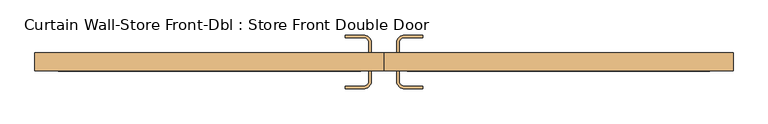
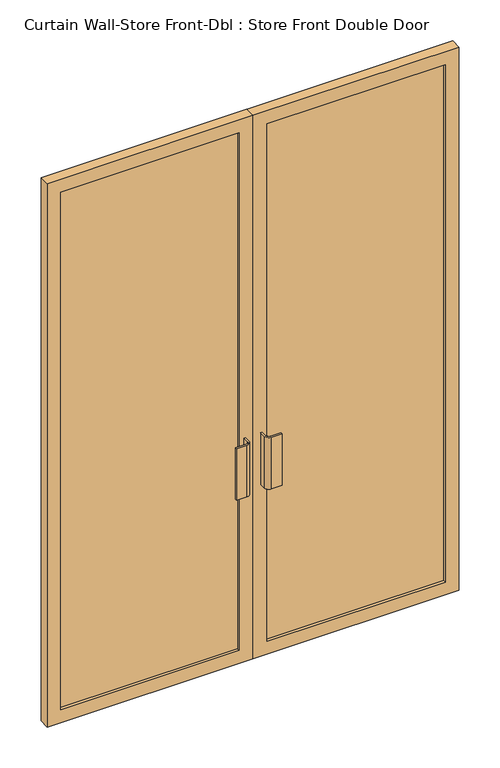
"""IFC4 building model written with IfcOpenShell, lengths in millimetres: door geometry, Curtain Wall-Store Front-Dbl : Store Front Double Door."""

import ifcopenshell
import ifcopenshell.guid

model = None  # the IFC model being written
_history = None  # IfcOwnerHistory: only IFC2X3 demands one
_inside = {}  # id of a spatial element -> (the spatial element, [elements in it])
_under = {}  # id of a project, library or spatial element -> (it, [spatial elements below it])
_declared = {}  # id of a project -> (the project, [libraries it declares])
_typed = {}  # id of a type object -> (the type object, [elements of that type])
_made_of = {}  # id of a material, layer set ... -> (it, [elements and type objects made of it])


def new_model(schema):
    """Start an empty IFC model of exactly this schema.

    Asked for "IFC4X3", IfcOpenShell would pick the latest addendum, in which some entities
    have other attributes; the version numbers below select the first issue.
    IFC2X3 requires an IfcOwnerHistory on every rooted entity: one is made here for all.
    """
    global model, _history
    if schema == "IFC4X3":
        model = ifcopenshell.file(schema_version=(4, 3, 0, 0))
    else:
        model = ifcopenshell.file(schema=schema)
    _inside.clear()
    _under.clear()
    _declared.clear()
    _typed.clear()
    _made_of.clear()
    _history = None
    if model.schema == "IFC2X3":
        org = make("IfcOrganization", Name="unknown")
        user = make(
            "IfcPersonAndOrganization",
            ThePerson=make("IfcPerson", FamilyName="unknown"),
            TheOrganization=org,
        )
        app = make(
            "IfcApplication",
            ApplicationDeveloper=org,
            Version="unknown",
            ApplicationFullName="unknown",
            ApplicationIdentifier="unknown",
        )
        _history = make(
            "IfcOwnerHistory",
            OwningUser=user,
            OwningApplication=app,
            ChangeAction="ADDED",
            CreationDate=0,
        )
    return model


def make(cls, **values):
    """One entity of the class cls with the attributes given. An attribute that is None is left unset."""
    return model.create_entity(
        cls, **{name: value for name, value in values.items() if value is not None}
    )


def rooted(cls, **values):
    """An entity with a GlobalId (a new one), such as an element, a storey or a relation."""
    return make(cls, GlobalId=ifcopenshell.guid.new(), OwnerHistory=_history, **values)


def si_unit(unit_type, name, prefix=None):
    """IfcSIUnit, for example si_unit("LENGTHUNIT", "METRE", prefix="MILLI")."""
    return make("IfcSIUnit", UnitType=unit_type, Prefix=prefix, Name=name)


def assignment(units):
    """IfcUnitAssignment: the units of a project."""
    return None if units is None else make("IfcUnitAssignment", Units=units)


def point(xyz):
    """IfcCartesianPoint."""
    return None if xyz is None else make("IfcCartesianPoint", Coordinates=xyz)


def direction(xyz):
    """IfcDirection."""
    return None if xyz is None else make("IfcDirection", DirectionRatios=xyz)


def frame(location, z_axis=None, x_axis=None):
    """IfcAxis2Placement3D, a coordinate frame: its origin and axes. An axis left out is left unset."""
    return make(
        "IfcAxis2Placement3D",
        Location=point(location),
        Axis=direction(z_axis),
        RefDirection=direction(x_axis),
    )


def frame_2d(location, x_axis=None):
    """IfcAxis2Placement2D, a coordinate frame in the plane: its origin and x axis."""
    return make(
        "IfcAxis2Placement2D", Location=point(location), RefDirection=direction(x_axis)
    )


def origin():
    """The frame at (0, 0, 0) with its axes left unset."""
    return frame((0.0, 0.0, 0.0))


def place(relative_to, where):
    """IfcLocalPlacement: puts the frame where relative to a parent placement (None: the world)."""
    return make(
        "IfcLocalPlacement", PlacementRelTo=relative_to, RelativePlacement=where
    )


def context(
    kind, dimensions, precision=None, world=None, true_north=None, identifier=None
):
    """IfcGeometricRepresentationContext, for example the 3D "Model" context."""
    return make(
        "IfcGeometricRepresentationContext",
        ContextIdentifier=identifier,
        ContextType=kind,
        CoordinateSpaceDimension=dimensions,
        Precision=precision,
        WorldCoordinateSystem=world,
        TrueNorth=true_north,
    )


def project(units=None, contexts=None):
    """IfcProject with its units and contexts."""
    return rooted(
        "IfcProject",
        Name="project",
        RepresentationContexts=contexts,
        UnitsInContext=assignment(units),
    )


def spatial(cls, under=None, at=None, **own):
    """A site, building, storey or space (cls), placed at a placement, below another one or the project."""
    s = rooted(cls, ObjectPlacement=at, **own)
    if under is not None:
        _under.setdefault(under.id(), (under, []))[1].append(s)
    return s


def polyline(points):
    """IfcPolyline through the points."""
    return make("IfcPolyline", Points=[point(p) for p in points])


def circle_curve(where, radius):
    """IfcCircle in the frame where."""
    return make("IfcCircle", Position=where, Radius=radius)


def trimmed(basis, trim1, trim2, sense, master):
    """IfcTrimmedCurve: the piece of a basis curve between two trims."""
    return make(
        "IfcTrimmedCurve",
        BasisCurve=basis,
        Trim1=trim1,
        Trim2=trim2,
        SenseAgreement=sense,
        MasterRepresentation=master,
    )


def segment(curve, same_sense, transition):
    """IfcCompositeCurveSegment."""
    return make(
        "IfcCompositeCurveSegment",
        Transition=transition,
        SameSense=same_sense,
        ParentCurve=curve,
    )


def composite_curve(segments, self_intersect=None):
    """IfcCompositeCurve: segments joined end to end."""
    return make("IfcCompositeCurve", Segments=segments, SelfIntersect=self_intersect)


def outline(outer, holes=None, kind="AREA"):
    """IfcArbitraryClosedProfileDef: a profile drawn as a closed curve; with holes, ...WithVoids."""
    if holes is None:
        return make("IfcArbitraryClosedProfileDef", ProfileType=kind, OuterCurve=outer)
    return make(
        "IfcArbitraryProfileDefWithVoids",
        ProfileType=kind,
        OuterCurve=outer,
        InnerCurves=holes,
    )


def extrude(swept, where, along, depth):
    """IfcExtrudedAreaSolid: the profile swept, set in the frame where, extruded along a direction by depth."""
    return make(
        "IfcExtrudedAreaSolid",
        SweptArea=swept,
        Position=where,
        ExtrudedDirection=direction(along),
        Depth=depth,
    )


def shape(context_of_items, identifier, shape_type, items):
    """IfcShapeRepresentation: the items that make up one representation, for example the "Body"."""
    return make(
        "IfcShapeRepresentation",
        ContextOfItems=context_of_items,
        RepresentationIdentifier=identifier,
        RepresentationType=shape_type,
        Items=items,
    )


def source(mapping_origin, context_of_items, identifier, shape_type, items):
    """IfcRepresentationMap: a shape defined once, which mapped items show again and again."""
    return make(
        "IfcRepresentationMap",
        MappingOrigin=mapping_origin,
        MappedRepresentation=shape(context_of_items, identifier, shape_type, items),
    )


def transform(
    local_origin,
    x_axis=None,
    y_axis=None,
    z_axis=None,
    scale=None,
    scale2=None,
    scale3=None,
    uniform=True,
):
    """IfcCartesianTransformationOperator3D, or its non-uniform kind. x_axis, y_axis, z_axis: its Axis1, 2, 3."""
    if uniform:
        return make(
            "IfcCartesianTransformationOperator3D",
            Axis1=direction(x_axis),
            Axis2=direction(y_axis),
            LocalOrigin=point(local_origin),
            Scale=scale,
            Axis3=direction(z_axis),
        )
    return make(
        "IfcCartesianTransformationOperator3DnonUniform",
        Axis1=direction(x_axis),
        Axis2=direction(y_axis),
        LocalOrigin=point(local_origin),
        Scale=scale,
        Axis3=direction(z_axis),
        Scale2=scale2,
        Scale3=scale3,
    )


def mapped(mapping_source, mapping_target):
    """IfcMappedItem: shows the shape of a source again, moved by a transform."""
    return make(
        "IfcMappedItem", MappingSource=mapping_source, MappingTarget=mapping_target
    )


def made_of(thing, what):
    """Note that an element or type object is made of a material, layer set ...; save() writes the relation."""
    if what is not None:
        _made_of.setdefault(what.id(), (what, []))[1].append(thing)
    return thing


def element(
    cls,
    number,
    at=None,
    inside=None,
    cuts=None,
    type_object=None,
    material=None,
    context=None,
    identifier="Body",
    shape_type=None,
    held_by="IfcProductDefinitionShape",
    body=None,
    shapes=None,
    **own,
):
    """One element of the class cls, such as IfcWall. Its Tag is "e" and its number.

    at: its placement. inside: the storey or other place that contains it. cuts: it is an
    opening in that element (IfcRelVoidsElement). A single representation is given by context,
    identifier, shape_type and body (its items); several are given by shapes. held_by: the class
    of the entity that holds the representations. save() writes the other relations.
    """
    e = rooted(cls, Tag="e%d" % number, ObjectPlacement=at, **own)
    if body is not None:
        shapes = [shape(context, identifier, shape_type, body)]
    if shapes is not None:
        e.Representation = make(held_by, Representations=shapes)
    if inside is not None:
        _inside.setdefault(inside.id(), (inside, []))[1].append(e)
    if cuts is not None:
        rooted(
            "IfcRelVoidsElement", RelatingBuildingElement=cuts, RelatedOpeningElement=e
        )
    if type_object is not None:
        _typed.setdefault(type_object.id(), (type_object, []))[1].append(e)
    return made_of(e, material)


def aggregate(whole, parts):
    """IfcRelAggregates: a whole, such as a stair, and the parts it consists of."""
    return rooted("IfcRelAggregates", RelatingObject=whole, RelatedObjects=parts)


def save(model, path):
    """Write the relations noted so far, then the file.

    IfcRelAggregates (storeys below a building ...), IfcRelContainedInSpatialStructure (elements
    in a storey), IfcRelDefinesByType, IfcRelAssociatesMaterial and IfcRelDeclares: one each for
    every whole, place, type object, material and project.
    """
    for whole, parts in _under.values():
        aggregate(whole, parts)
    for where, things in _inside.values():
        rooted(
            "IfcRelContainedInSpatialStructure",
            RelatedElements=things,
            RelatingStructure=where,
        )
    for kind, things in _typed.values():
        rooted("IfcRelDefinesByType", RelatedObjects=things, RelatingType=kind)
    for what, things in _made_of.values():
        rooted("IfcRelAssociatesMaterial", RelatedObjects=things, RelatingMaterial=what)
    for by, libraries in _declared.values():
        rooted("IfcRelDeclares", RelatingContext=by, RelatedDefinitions=libraries)
    model.write(path)


def curtain_wall_store_front_dbl_store_front_double_door_6ddc461a(model_context):
    return source(origin(), model_context, "Body", "SweptSolid", [
        extrude(outline(composite_curve([segment(polyline([(-31.75, 12.7), (-31.75, -12.7), (-38.1, -12.7), (-38.1, 12.7)]), True, "CONTINUOUS"), segment(trimmed(circle_curve(frame_2d((-50.8, 12.7)), 12.7), [point((-38.1, 12.7))], [point((-50.8, 25.4))], True, "CARTESIAN"), True, "CONTINUOUS"), segment(polyline([(-50.8, 25.4), (-95.25, 25.4), (-95.25, 31.75), (-50.8, 31.75)]), True, "CONTINUOUS"), segment(trimmed(circle_curve(frame_2d((-50.8, 12.7)), 19.05), [point((-50.8, 31.75))], [point((-31.75, 12.7))], False, "CARTESIAN"), True, "CONTINUOUS")], self_intersect=False)), frame((0.0, 0.0, 762.0), z_axis=(0.0, 0.0, 1.0), x_axis=(1.0, 0.0, 0.0)), (0.0, 0.0, 1.0), 228.6),
        extrude(outline(composite_curve([segment(trimmed(circle_curve(frame_2d((50.8, 12.7)), 19.05), [point((31.75, 12.7))], [point((50.8, 31.75))], False, "CARTESIAN"), True, "CONTINUOUS"), segment(polyline([(50.8, 31.75), (95.25, 31.75), (95.25, 25.4), (50.8, 25.4)]), True, "CONTINUOUS"), segment(trimmed(circle_curve(frame_2d((50.8, 12.7)), 12.7), [point((50.8, 25.4))], [point((38.1, 12.7))], True, "CARTESIAN"), True, "CONTINUOUS"), segment(polyline([(38.1, 12.7), (38.1, -12.7), (31.75, -12.7), (31.75, 12.7)]), True, "CONTINUOUS")], self_intersect=False)), frame((0.0, 0.0, 762.0), z_axis=(0.0, 0.0, 1.0), x_axis=(1.0, 0.0, 0.0)), (0.0, 0.0, 1.0), 228.6),
        extrude(outline(composite_curve([segment(trimmed(circle_curve(frame_2d((-50.8, -82.55)), 19.05), [point((-31.75, -82.55))], [point((-50.8, -101.6))], False, "CARTESIAN"), True, "CONTINUOUS"), segment(polyline([(-50.8, -101.6), (-95.25, -101.6), (-95.25, -95.25), (-50.8, -95.25)]), True, "CONTINUOUS"), segment(trimmed(circle_curve(frame_2d((-50.8, -82.55)), 12.7), [point((-50.8, -95.25))], [point((-38.1, -82.55))], True, "CARTESIAN"), True, "CONTINUOUS"), segment(polyline([(-38.1, -82.55), (-38.1, -57.15), (-31.75, -57.15), (-31.75, -82.55)]), True, "CONTINUOUS")], self_intersect=False)), frame((0.0, 0.0, 762.0), z_axis=(0.0, 0.0, 1.0), x_axis=(1.0, 0.0, 0.0)), (0.0, 0.0, 1.0), 228.6),
        extrude(outline(composite_curve([segment(polyline([(31.75, -82.55), (31.75, -57.15), (38.1, -57.15), (38.1, -82.55)]), True, "CONTINUOUS"), segment(trimmed(circle_curve(frame_2d((50.8, -82.55)), 12.7), [point((38.1, -82.55))], [point((50.8, -95.25))], True, "CARTESIAN"), True, "CONTINUOUS"), segment(polyline([(50.8, -95.25), (95.25, -95.25), (95.25, -101.6), (50.8, -101.6)]), True, "CONTINUOUS"), segment(trimmed(circle_curve(frame_2d((50.8, -82.55)), 19.05), [point((50.8, -101.6))], [point((31.75, -82.55))], False, "CARTESIAN"), True, "CONTINUOUS")], self_intersect=False)), frame((0.0, 0.0, 762.0), z_axis=(0.0, 0.0, 1.0), x_axis=(1.0, 0.0, 0.0)), (0.0, 0.0, 1.0), 228.6),
        extrude(outline(polyline([(806.45, -25.4), (806.45, -44.45), (57.94375, -44.45), (57.94375, -25.4), (806.45, -25.4)])), frame((0.0, 0.0, 57.15), z_axis=(0.0, 0.0, 1.0), x_axis=(1.0, 0.0, 0.0)), (0.0, 0.0, 1.0), 2292.35),
        extrude(outline(polyline([(-57.94375, -25.4), (-57.94375, -44.45), (-806.45, -44.45), (-806.45, -25.4), (-57.94375, -25.4)])), frame((0.0, 0.0, 57.15), z_axis=(0.0, 0.0, 1.0), x_axis=(1.0, 0.0, 0.0)), (0.0, 0.0, 1.0), 2292.35),
        extrude(outline(polyline([(2406.65, 0.79375), (0.0, 0.79375), (0.0, 863.6), (2406.65, 863.6), (2406.65, 0.79375)]), holes=[polyline([(2349.5, 57.94375), (2349.5, 806.45), (57.15, 806.45), (57.15, 57.94375), (2349.5, 57.94375)])]), frame((0.0, -57.15, 0.0), z_axis=(0.0, 1.0, 0.0), x_axis=(0.0, 0.0, 1.0)), (0.0, 0.0, 1.0), 44.45),
        extrude(outline(polyline([(2406.65, -0.79375), (2406.65, -863.6), (0.0, -863.6), (0.0, -0.79375), (2406.65, -0.79375)]), holes=[polyline([(2349.5, -806.45), (2349.5, -57.94375), (57.15, -57.94375), (57.15, -806.45), (2349.5, -806.45)])]), frame((0.0, -57.15, 0.0), z_axis=(0.0, 1.0, 0.0), x_axis=(0.0, 0.0, 1.0)), (0.0, 0.0, 1.0), 44.45),
    ])


if __name__ == "__main__":
    model = new_model("IFC4")
    model_context = context("Model", 3, world=origin())
    ifc_project = project(units=[si_unit("LENGTHUNIT", "METRE", prefix="MILLI")], contexts=[model_context])
    site = spatial("IfcSite", under=ifc_project)
    building = spatial("IfcBuilding", under=site)
    placement = place(None, origin())
    curtain_wall_store_front_dbl_store_front_double_door_shape = curtain_wall_store_front_dbl_store_front_double_door_6ddc461a(model_context)
    element("IfcDoor", 1, ObjectType="Curtain Wall-Store Front-Dbl : Store Front Double Door", at=placement, inside=building, context=model_context, shape_type="MappedRepresentation", body=[
        mapped(curtain_wall_store_front_dbl_store_front_double_door_shape, transform((0.0, 0.0, 0.0), x_axis=(1.0, 0.0, 0.0), y_axis=(0.0, 1.0, 0.0), z_axis=(0.0, 0.0, 1.0))),
    ])
    save(model, "model.ifc")

# Revit data of these elements
# Type "Curtain Wall-Store Front-Dbl : Store Front Double Door"
#   Type Mark = "13"
#   Construction Type Id = "MDOOR"
#   Assembly Code = "B2030110"
#   Analytic Construction = "Metal"
#   Offset = 0' - 2 1/4"
#   Heat Transfer Coefficient (U) = 0.651978 BTU/(h·ft²·°F)
#   Define Thermal Properties by = 1
#   Define Thermal Properties by = 1
#   Function = 1
#   Material = Aluminum
#   Glazing Material = Glass
#   Visual Light Transmittance = 0
#   Solar Heat Gain Coefficient = 0
# Element 1 (IfcDoor, "Curtain Wall-Store Front-Dbl : Store Front Double Door")
#   Materials on its faces: "Aluminum", "Glass"
# Materials
#   "Aluminum": class "Metal", colour RGB 247 247 247, transparency 0, Description = "Aluminum 6061", Cost = 0
#   "Glass": class "Glass", colour RGB 0 128 192, transparency 0.75, Description = "Soda Lime Glass", Cost = 0
